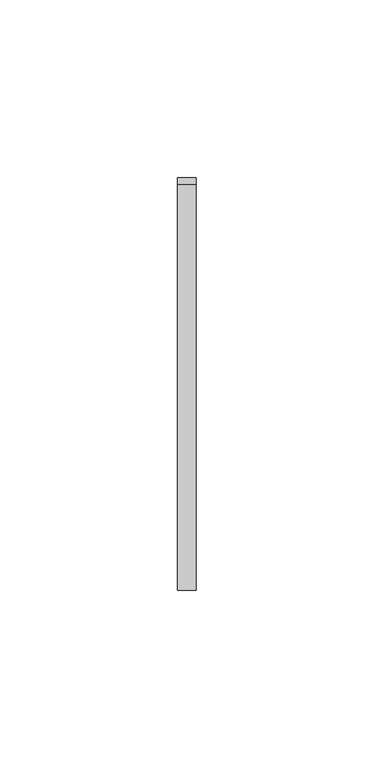
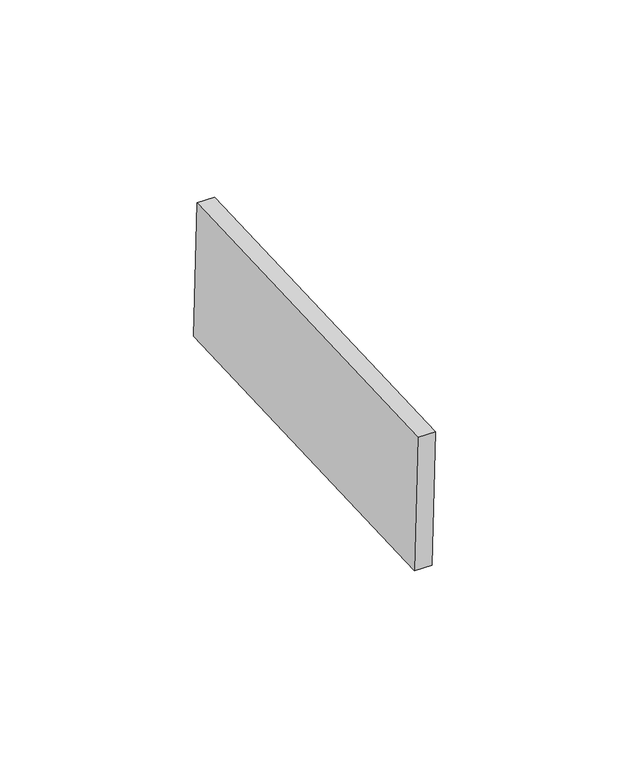
"""IFC4 building model written with IfcOpenShell, lengths in millimetres: proxy geometry, Inner panel:Inner panel:1:Inner panel:1 : Inner panel:Inner panel:300324:2:Inner panel:1:Inner panel:1 : Inner panel:Inner panel:300324:2 : Inner panel:Inner panel:1:Inner panel:1 : Inner panel:Inner panel:300324:300043:86 : Inner panel:Inner panel:1:Inner panel:1 : Inner panel:Inner panel:300324:2:Inner panel:1:Inner panel:1 : Inner panel:Inner panel:300324:2 : Inner panel:Inner panel:1:Inner panel:1 : Inner panel:Inner panel:300324:300043:308120."""

from ifc_helpers import new_model, si_unit, frame, origin, place, context, project, spatial, polyline, outline, extrude, source, transform, mapped, element, save


def generic_models_0dcdc921(model_context):
    return source(origin(), model_context, "Body", "SweptSolid", [
        extrude(outline(polyline([(0.0, -114.2999999), (0.0, 0.0), (5.2138089, 0.0), (5.2138089, -114.2999999), (0.0, -114.2999999)])), frame((592310.995117, -576618.8219505, 4051.6214343), z_axis=(0.0, -0.04163054471216399, 0.9991330730923527), x_axis=(-1.0, 0.0, 0.0)), (0.0, 0.0, 1.0), 43.2233908),
    ])


if __name__ == "__main__":
    model = new_model("IFC4")
    model_context = context("Model", 3, world=origin())
    ifc_project = project(units=[si_unit("LENGTHUNIT", "METRE", prefix="MILLI")], contexts=[model_context])
    site = spatial("IfcSite", under=ifc_project)
    building = spatial("IfcBuilding", under=site)
    placement = place(None, origin())
    generic_models_shape = generic_models_0dcdc921(model_context)
    element("IfcBuildingElementProxy", 1, Name="Inner panel:Inner panel:1:Inner panel:1 : Inner panel:Inner panel:300324:2:Inner panel:1:Inner panel:1 : Inner panel:Inner panel:300324:2 : Inner panel:Inner panel:1:Inner panel:1 : Inner panel:Inner panel:300324:300043:86 : Inner panel:Inner panel:1:Inner panel:1 : Inner panel:Inner panel:300324:2:Inner panel:1:Inner panel:1 : Inner panel:Inner panel:300324:2 : Inner panel:Inner panel:1:Inner panel:1 : Inner panel:Inner panel:300324:300043:308120", ObjectType="Inner panel:Inner panel:1:Inner panel:1 : Inner panel:Inner panel:300324:2:Inner panel:1:Inner panel:1 : Inner panel:Inner panel:300324:2 : Inner panel:Inner panel:1:Inner panel:1 : Inner panel:Inner panel:300324:300043:86 : Inner panel:Inner panel:1:Inner panel:1 : Inner panel:Inner panel:300324:2:Inner panel:1:Inner panel:1 : Inner panel:Inner panel:300324:2 : Inner panel:Inner panel:1:Inner panel:1 : Inner panel:Inner panel:300324:300043:308120", at=placement, inside=building, context=model_context, shape_type="MappedRepresentation", body=[
        mapped(generic_models_shape, transform((0.0, 0.0, 0.0), x_axis=(1.0, 0.0, 0.0), y_axis=(0.0, 1.0, 0.0), z_axis=(0.0, 0.0, 1.0))),
    ])
    save(model, "model.ifc")

# Revit data of these elements
# Type "Inner panel:Inner panel:1:Inner panel:1 : Inner panel:Inner panel:300324:2:Inner panel:1:Inner panel:1 : Inner panel:Inner panel:300324:2 : Inner panel:Inner panel:1:Inner panel:1 : Inner panel:Inner panel:300324:300043:86 : Inner panel:Inner panel:1:Inner panel:1 : Inner panel:Inner panel:300324:2:Inner panel:1:Inner panel:1 : Inner panel:Inner panel:300324:2 : Inner panel:Inner panel:1:Inner panel:1 : Inner panel:Inner panel:300324:300043:308120"
#   NameOverride = "Inner panel:Inner panel:1:Inner panel:1 : Inner panel:Inner panel:300324:2:Inner panel:1:Inner panel:1 : Inner panel:Inner panel:300324:2 : Inner panel:Inner panel:1:Inner panel:1 : Inner panel:Inner panel:300324:300043:308120"
#   ObjectTypeOverride = "Inner panel:1:Inner panel:1 : Inner panel:Inner panel:300324:2 : Inner panel:Inner panel:1:Inner panel:1 : Inner panel:Inner panel:300324:300043"
#   Reference = "Inner panel"
#   Tag = "308120"
# Element 1 (IfcBuildingElementProxy, "Inner panel:Inner panel:1:Inner panel:1 : Inner panel:Inner panel:300324:2:Inner panel:1:Inner panel:1 : Inner panel:Inner panel:300324:2 : Inner panel:Inner panel:1:Inner panel:1 : Inner panel:Inner panel:300324:300043:86 : Inner panel:Inner panel:1:Inner panel:1 : Inner panel:Inner panel:300324:2:Inner panel:1:Inner panel:1 : Inner panel:Inner panel:300324:2 : Inner panel:Inner panel:1:Inner panel:1 : Inner panel:Inner panel:300324:300043:308120")
#   Materials on its faces: "SLIDING CLIP"
# Materials
#   "SLIDING CLIP": class "Generic", colour RGB 120 120 120, transparency 0, Cost = 0
